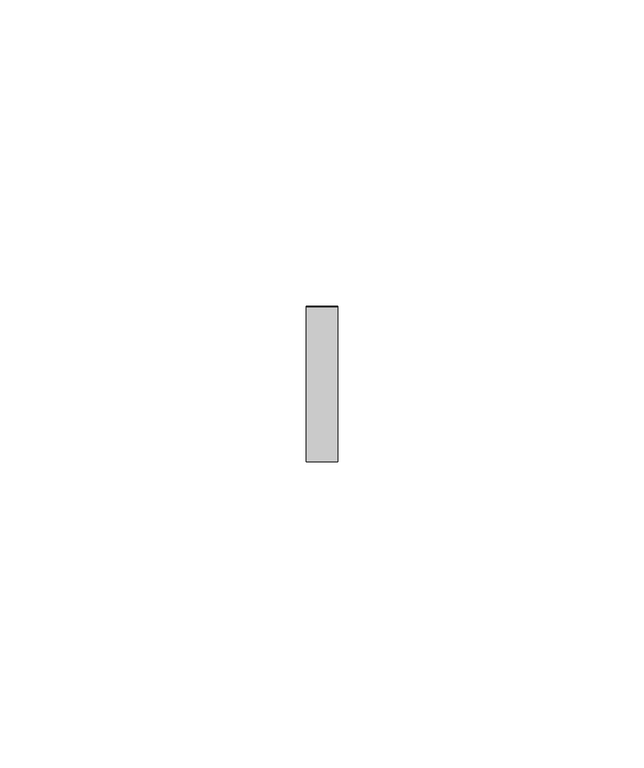
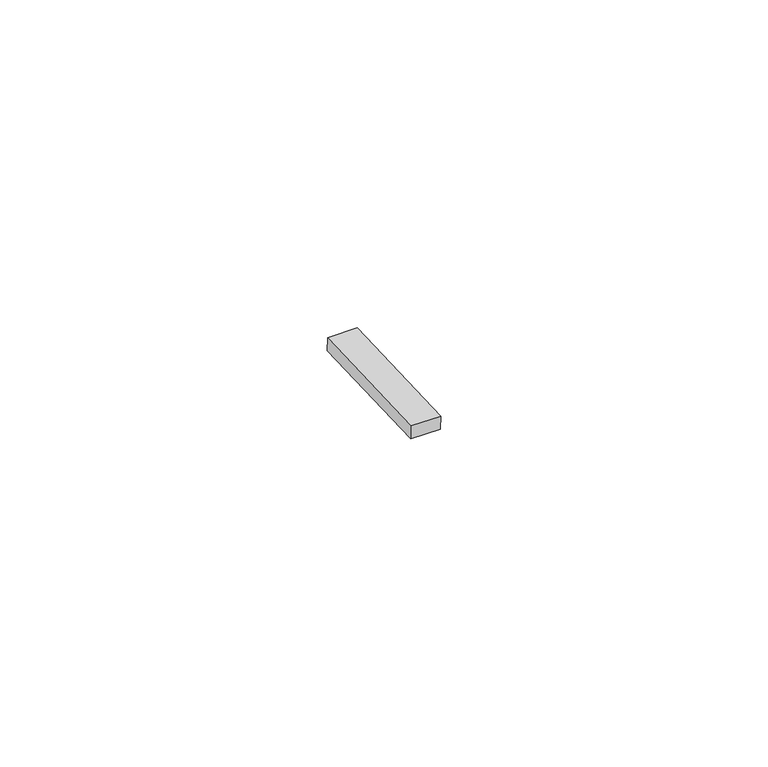
"""IFC4 building model written with IfcOpenShell, lengths in millimetres: proxy geometry, Inner panel:Inner panel:1:Inner panel:1 : Inner panel:Inner panel:300324:2:Inner panel:1:Inner panel:1 : Inner panel:Inner panel:300324:2 : Inner panel:Inner panel:1:Inner panel:1 : Inner panel:Inner panel:300324:300043:121 : Inner panel:Inner panel:1:Inner panel:1 : Inner panel:Inner panel:300324:2:Inner panel:1:Inner panel:1 : Inner panel:Inner panel:300324:2 : Inner panel:Inner panel:1:Inner panel:1 : Inner panel:Inner panel:300324:300043:308120."""

from ifc_helpers import new_model, si_unit, frame, origin, place, context, project, spatial, polyline, outline, extrude, source, transform, mapped, element, save


def generic_models_5b28e56e(model_context):
    return source(origin(), model_context, "Body", "SweptSolid", [
        extrude(outline(polyline([(0.0, -25.3999999), (0.0, 0.0), (5.2138089, 0.0), (5.2138089, -25.3999999), (0.0, -25.3999999)])), frame((591904.595117, -578962.7476805, 3951.4793391), z_axis=(0.0, -0.041630544712223896, 0.9991330730923502), x_axis=(-1.0, 0.0, 0.0)), (0.0, 0.0, 1.0), 2.4763745),
    ])


if __name__ == "__main__":
    model = new_model("IFC4")
    model_context = context("Model", 3, world=origin())
    ifc_project = project(units=[si_unit("LENGTHUNIT", "METRE", prefix="MILLI")], contexts=[model_context])
    site = spatial("IfcSite", under=ifc_project)
    building = spatial("IfcBuilding", under=site)
    placement = place(None, origin())
    generic_models_shape = generic_models_5b28e56e(model_context)
    element("IfcBuildingElementProxy", 1, Name="Inner panel:Inner panel:1:Inner panel:1 : Inner panel:Inner panel:300324:2:Inner panel:1:Inner panel:1 : Inner panel:Inner panel:300324:2 : Inner panel:Inner panel:1:Inner panel:1 : Inner panel:Inner panel:300324:300043:121 : Inner panel:Inner panel:1:Inner panel:1 : Inner panel:Inner panel:300324:2:Inner panel:1:Inner panel:1 : Inner panel:Inner panel:300324:2 : Inner panel:Inner panel:1:Inner panel:1 : Inner panel:Inner panel:300324:300043:308120", ObjectType="Inner panel:Inner panel:1:Inner panel:1 : Inner panel:Inner panel:300324:2:Inner panel:1:Inner panel:1 : Inner panel:Inner panel:300324:2 : Inner panel:Inner panel:1:Inner panel:1 : Inner panel:Inner panel:300324:300043:121 : Inner panel:Inner panel:1:Inner panel:1 : Inner panel:Inner panel:300324:2:Inner panel:1:Inner panel:1 : Inner panel:Inner panel:300324:2 : Inner panel:Inner panel:1:Inner panel:1 : Inner panel:Inner panel:300324:300043:308120", at=placement, inside=building, context=model_context, shape_type="MappedRepresentation", body=[
        mapped(generic_models_shape, transform((0.0, 0.0, 0.0), x_axis=(1.0, 0.0, 0.0), y_axis=(0.0, 1.0, 0.0), z_axis=(0.0, 0.0, 1.0))),
    ])
    save(model, "model.ifc")

# Revit data of these elements
# Type "Inner panel:Inner panel:1:Inner panel:1 : Inner panel:Inner panel:300324:2:Inner panel:1:Inner panel:1 : Inner panel:Inner panel:300324:2 : Inner panel:Inner panel:1:Inner panel:1 : Inner panel:Inner panel:300324:300043:121 : Inner panel:Inner panel:1:Inner panel:1 : Inner panel:Inner panel:300324:2:Inner panel:1:Inner panel:1 : Inner panel:Inner panel:300324:2 : Inner panel:Inner panel:1:Inner panel:1 : Inner panel:Inner panel:300324:300043:308120"
#   NameOverride = "Inner panel:Inner panel:1:Inner panel:1 : Inner panel:Inner panel:300324:2:Inner panel:1:Inner panel:1 : Inner panel:Inner panel:300324:2 : Inner panel:Inner panel:1:Inner panel:1 : Inner panel:Inner panel:300324:300043:308120"
#   ObjectTypeOverride = "Inner panel:1:Inner panel:1 : Inner panel:Inner panel:300324:2 : Inner panel:Inner panel:1:Inner panel:1 : Inner panel:Inner panel:300324:300043"
#   Reference = "Inner panel"
#   Tag = "308120"
# Element 1 (IfcBuildingElementProxy, "Inner panel:Inner panel:1:Inner panel:1 : Inner panel:Inner panel:300324:2:Inner panel:1:Inner panel:1 : Inner panel:Inner panel:300324:2 : Inner panel:Inner panel:1:Inner panel:1 : Inner panel:Inner panel:300324:300043:121 : Inner panel:Inner panel:1:Inner panel:1 : Inner panel:Inner panel:300324:2:Inner panel:1:Inner panel:1 : Inner panel:Inner panel:300324:2 : Inner panel:Inner panel:1:Inner panel:1 : Inner panel:Inner panel:300324:300043:308120")
#   Materials on its faces: "AT CLIP - 1\" WIDE NON ABSORBENT, WEATHER-RESISTANT NEOPRENE/EPDM/SBR FOAM"
# Materials
#   "AT CLIP - 1\" WIDE NON ABSORBENT, WEATHER-RESISTANT NEOPRENE/EPDM/SBR FOAM": class "Generic", colour RGB 85 85 85, transparency 0, Cost = 0
